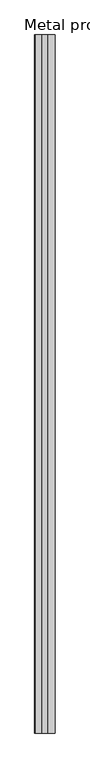
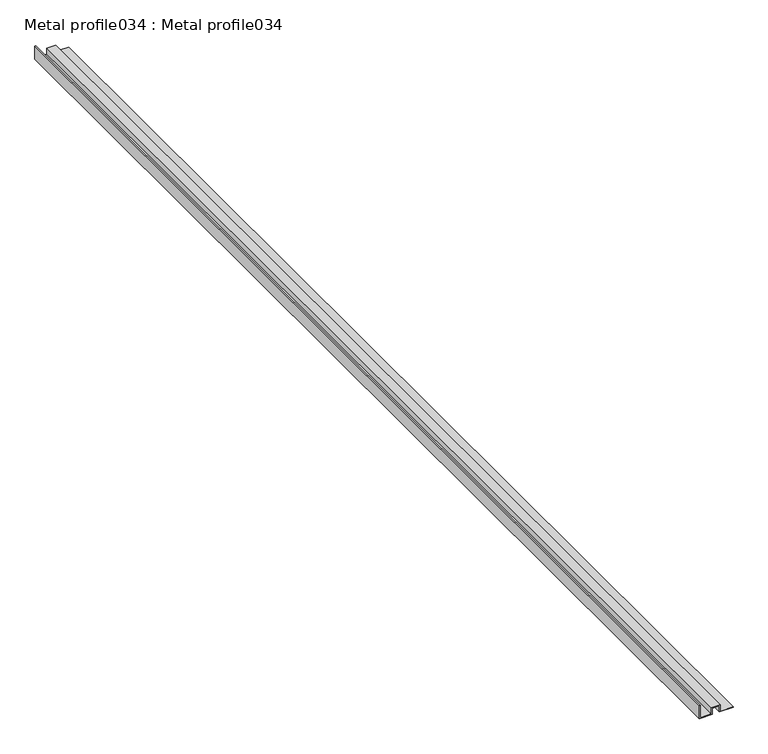
"""IFC4 building model written with IfcOpenShell, lengths in millimetres: proxy geometry, Metal profile034 : Metal profile034."""

from ifc_helpers import new_model, si_unit, frame, origin, place, context, project, spatial, polyline, outline, extrude, source, transform, mapped, element, save


def metal_profile034_metal_profile034_580b1cdc(model_context):
    return source(origin(), model_context, "Body", "SweptSolid", [
        extrude(outline(polyline([(39543.8875708, -7249.6295075), (39543.8875708, -7227.4045075), (39555.3175708, -7227.4045075), (39555.3175708, -7214.7045075), (39543.8875708, -7214.7045075), (39543.8875708, -7190.9913235), (39545.1675708, -7190.9913235), (39545.1675708, -7213.4245075), (39556.5975708, -7213.4245075), (39556.5975708, -7228.6845075), (39545.1675708, -7228.6845075), (39545.1675708, -7248.3495075), (39567.6883323, -7248.3495075), (39567.6883323, -7249.6295075), (39543.8875708, -7249.6295075)])), frame((0.0, 7982.1531721, 0.0), z_axis=(0.0, 1.0, 0.0), x_axis=(0.0, 0.0, 1.0)), (0.0, 0.0, 1.0), 2000.0),
    ])


if __name__ == "__main__":
    model = new_model("IFC4")
    model_context = context("Model", 3, world=origin())
    ifc_project = project(units=[si_unit("LENGTHUNIT", "METRE", prefix="MILLI")], contexts=[model_context])
    site = spatial("IfcSite", under=ifc_project)
    building = spatial("IfcBuilding", under=site)
    placement = place(None, origin())
    metal_profile034_metal_profile034_shape = metal_profile034_metal_profile034_580b1cdc(model_context)
    element("IfcBuildingElementProxy", 1, Name="Metal profile034 : Metal profile034", ObjectType="Metal profile034 : Metal profile034", at=placement, inside=building, context=model_context, shape_type="MappedRepresentation", body=[
        mapped(metal_profile034_metal_profile034_shape, transform((0.0, 0.0, 0.0), x_axis=(1.0, 0.0, 0.0), y_axis=(0.0, 1.0, 0.0), z_axis=(0.0, 0.0, 1.0))),
    ])
    save(model, "model.ifc")

# Revit data of these elements
# Type "Metal profile034 : Metal profile034"
#   NameOverride = "Metal profile034"
# Element 1 (IfcBuildingElementProxy, "Metal profile034 : Metal profile034")
#   Materials on its faces: "16 GA. COPPER SOFFIT DRIP SCREED"
# Materials
#   "16 GA. COPPER SOFFIT DRIP SCREED": class "Unassigned", colour RGB 255 217 0, transparency 0
